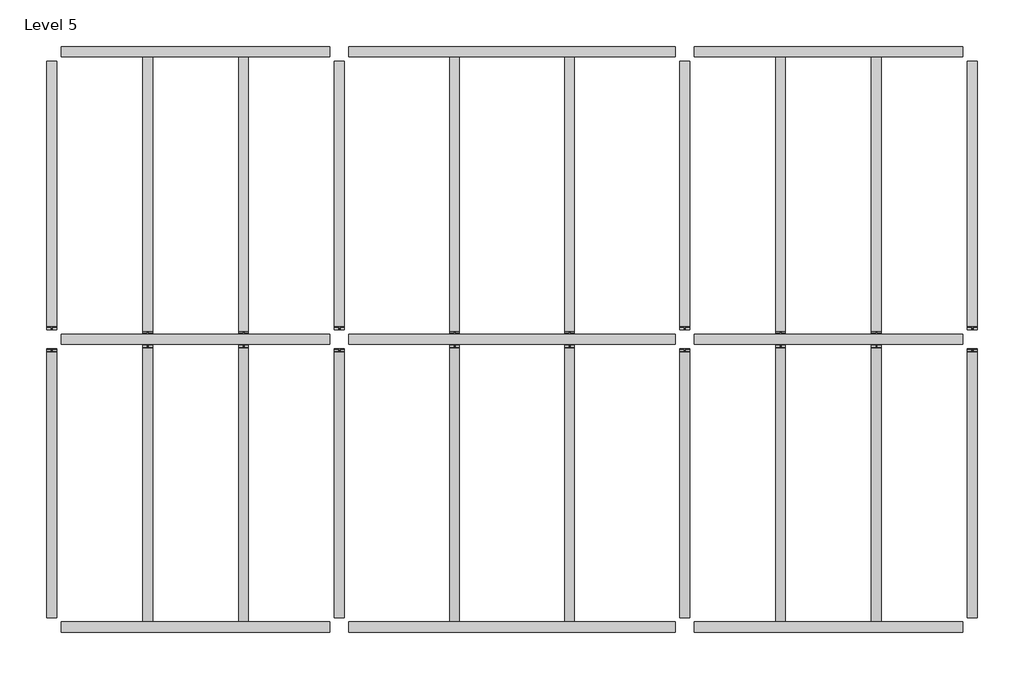
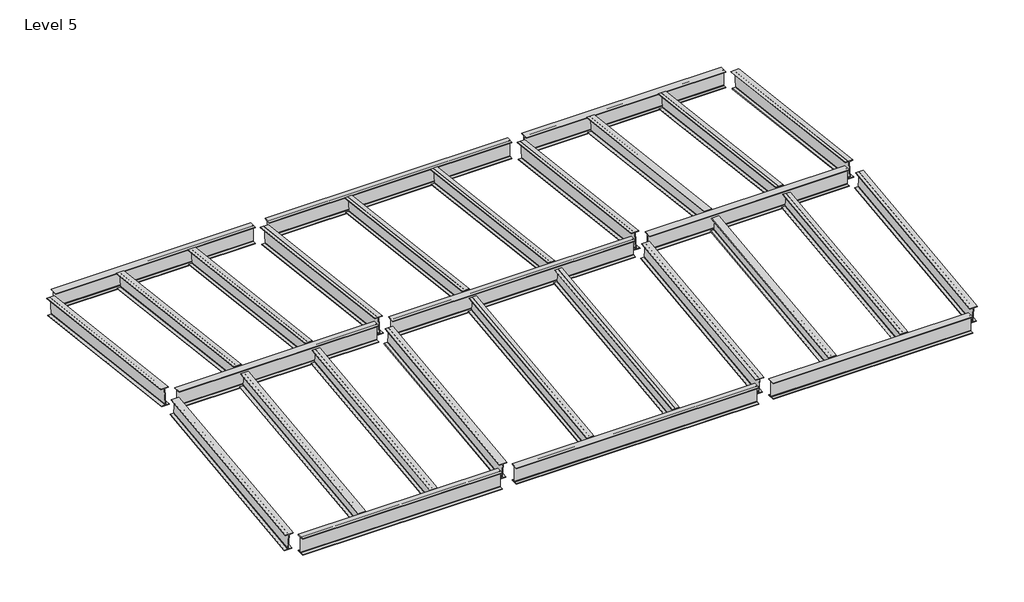
# One storey: 29 beams.
"""IFC4 building model written with IfcOpenShell, lengths in millimetres."""

import ifcopenshell
import ifcopenshell.guid

model = None  # the IFC model being written
_history = None  # IfcOwnerHistory: only IFC2X3 demands one
_inside = {}  # id of a spatial element -> (the spatial element, [elements in it])
_under = {}  # id of a project, library or spatial element -> (it, [spatial elements below it])
_declared = {}  # id of a project -> (the project, [libraries it declares])
_typed = {}  # id of a type object -> (the type object, [elements of that type])
_made_of = {}  # id of a material, layer set ... -> (it, [elements and type objects made of it])


def new_model(schema):
    """Start an empty IFC model of exactly this schema.

    Asked for "IFC4X3", IfcOpenShell would pick the latest addendum, in which some entities
    have other attributes; the version numbers below select the first issue.
    IFC2X3 requires an IfcOwnerHistory on every rooted entity: one is made here for all.
    """
    global model, _history
    if schema == "IFC4X3":
        model = ifcopenshell.file(schema_version=(4, 3, 0, 0))
    else:
        model = ifcopenshell.file(schema=schema)
    _inside.clear()
    _under.clear()
    _declared.clear()
    _typed.clear()
    _made_of.clear()
    _history = None
    if model.schema == "IFC2X3":
        org = make("IfcOrganization", Name="unknown")
        user = make(
            "IfcPersonAndOrganization",
            ThePerson=make("IfcPerson", FamilyName="unknown"),
            TheOrganization=org,
        )
        app = make(
            "IfcApplication",
            ApplicationDeveloper=org,
            Version="unknown",
            ApplicationFullName="unknown",
            ApplicationIdentifier="unknown",
        )
        _history = make(
            "IfcOwnerHistory",
            OwningUser=user,
            OwningApplication=app,
            ChangeAction="ADDED",
            CreationDate=0,
        )
    return model


def make(cls, **values):
    """One entity of the class cls with the attributes given. An attribute that is None is left unset."""
    return model.create_entity(
        cls, **{name: value for name, value in values.items() if value is not None}
    )


def rooted(cls, **values):
    """An entity with a GlobalId (a new one), such as an element, a storey or a relation."""
    return make(cls, GlobalId=ifcopenshell.guid.new(), OwnerHistory=_history, **values)


def si_unit(unit_type, name, prefix=None):
    """IfcSIUnit, for example si_unit("LENGTHUNIT", "METRE", prefix="MILLI")."""
    return make("IfcSIUnit", UnitType=unit_type, Prefix=prefix, Name=name)


def assignment(units):
    """IfcUnitAssignment: the units of a project."""
    return None if units is None else make("IfcUnitAssignment", Units=units)


def point(xyz):
    """IfcCartesianPoint."""
    return None if xyz is None else make("IfcCartesianPoint", Coordinates=xyz)


def direction(xyz):
    """IfcDirection."""
    return None if xyz is None else make("IfcDirection", DirectionRatios=xyz)


def frame(location, z_axis=None, x_axis=None):
    """IfcAxis2Placement3D, a coordinate frame: its origin and axes. An axis left out is left unset."""
    return make(
        "IfcAxis2Placement3D",
        Location=point(location),
        Axis=direction(z_axis),
        RefDirection=direction(x_axis),
    )


def frame_2d(location, x_axis=None):
    """IfcAxis2Placement2D, a coordinate frame in the plane: its origin and x axis."""
    return make(
        "IfcAxis2Placement2D", Location=point(location), RefDirection=direction(x_axis)
    )


def origin():
    """The frame at (0, 0, 0) with its axes left unset."""
    return frame((0.0, 0.0, 0.0))


def place(relative_to, where):
    """IfcLocalPlacement: puts the frame where relative to a parent placement (None: the world)."""
    return make(
        "IfcLocalPlacement", PlacementRelTo=relative_to, RelativePlacement=where
    )


def context(
    kind, dimensions, precision=None, world=None, true_north=None, identifier=None
):
    """IfcGeometricRepresentationContext, for example the 3D "Model" context."""
    return make(
        "IfcGeometricRepresentationContext",
        ContextIdentifier=identifier,
        ContextType=kind,
        CoordinateSpaceDimension=dimensions,
        Precision=precision,
        WorldCoordinateSystem=world,
        TrueNorth=true_north,
    )


def project(units=None, contexts=None):
    """IfcProject with its units and contexts."""
    return rooted(
        "IfcProject",
        Name="project",
        RepresentationContexts=contexts,
        UnitsInContext=assignment(units),
    )


def spatial(cls, under=None, at=None, **own):
    """A site, building, storey or space (cls), placed at a placement, below another one or the project."""
    s = rooted(cls, ObjectPlacement=at, **own)
    if under is not None:
        _under.setdefault(under.id(), (under, []))[1].append(s)
    return s


def polyline(points):
    """IfcPolyline through the points."""
    return make("IfcPolyline", Points=[point(p) for p in points])


def circle_curve(where, radius):
    """IfcCircle in the frame where."""
    return make("IfcCircle", Position=where, Radius=radius)


def trimmed(basis, trim1, trim2, sense, master):
    """IfcTrimmedCurve: the piece of a basis curve between two trims."""
    return make(
        "IfcTrimmedCurve",
        BasisCurve=basis,
        Trim1=trim1,
        Trim2=trim2,
        SenseAgreement=sense,
        MasterRepresentation=master,
    )


def segment(curve, same_sense, transition):
    """IfcCompositeCurveSegment."""
    return make(
        "IfcCompositeCurveSegment",
        Transition=transition,
        SameSense=same_sense,
        ParentCurve=curve,
    )


def composite_curve(segments, self_intersect=None):
    """IfcCompositeCurve: segments joined end to end."""
    return make("IfcCompositeCurve", Segments=segments, SelfIntersect=self_intersect)


def outline(outer, holes=None, kind="AREA"):
    """IfcArbitraryClosedProfileDef: a profile drawn as a closed curve; with holes, ...WithVoids."""
    if holes is None:
        return make("IfcArbitraryClosedProfileDef", ProfileType=kind, OuterCurve=outer)
    return make(
        "IfcArbitraryProfileDefWithVoids",
        ProfileType=kind,
        OuterCurve=outer,
        InnerCurves=holes,
    )


def extrude(swept, where, along, depth):
    """IfcExtrudedAreaSolid: the profile swept, set in the frame where, extruded along a direction by depth."""
    return make(
        "IfcExtrudedAreaSolid",
        SweptArea=swept,
        Position=where,
        ExtrudedDirection=direction(along),
        Depth=depth,
    )


def shape(context_of_items, identifier, shape_type, items):
    """IfcShapeRepresentation: the items that make up one representation, for example the "Body"."""
    return make(
        "IfcShapeRepresentation",
        ContextOfItems=context_of_items,
        RepresentationIdentifier=identifier,
        RepresentationType=shape_type,
        Items=items,
    )


def source(mapping_origin, context_of_items, identifier, shape_type, items):
    """IfcRepresentationMap: a shape defined once, which mapped items show again and again."""
    return make(
        "IfcRepresentationMap",
        MappingOrigin=mapping_origin,
        MappedRepresentation=shape(context_of_items, identifier, shape_type, items),
    )


def transform(
    local_origin,
    x_axis=None,
    y_axis=None,
    z_axis=None,
    scale=None,
    scale2=None,
    scale3=None,
    uniform=True,
):
    """IfcCartesianTransformationOperator3D, or its non-uniform kind. x_axis, y_axis, z_axis: its Axis1, 2, 3."""
    if uniform:
        return make(
            "IfcCartesianTransformationOperator3D",
            Axis1=direction(x_axis),
            Axis2=direction(y_axis),
            LocalOrigin=point(local_origin),
            Scale=scale,
            Axis3=direction(z_axis),
        )
    return make(
        "IfcCartesianTransformationOperator3DnonUniform",
        Axis1=direction(x_axis),
        Axis2=direction(y_axis),
        LocalOrigin=point(local_origin),
        Scale=scale,
        Axis3=direction(z_axis),
        Scale2=scale2,
        Scale3=scale3,
    )


def mapped(mapping_source, mapping_target):
    """IfcMappedItem: shows the shape of a source again, moved by a transform."""
    return make(
        "IfcMappedItem", MappingSource=mapping_source, MappingTarget=mapping_target
    )


def made_of(thing, what):
    """Note that an element or type object is made of a material, layer set ...; save() writes the relation."""
    if what is not None:
        _made_of.setdefault(what.id(), (what, []))[1].append(thing)
    return thing


def element(
    cls,
    number,
    at=None,
    inside=None,
    cuts=None,
    type_object=None,
    material=None,
    context=None,
    identifier="Body",
    shape_type=None,
    held_by="IfcProductDefinitionShape",
    body=None,
    shapes=None,
    **own,
):
    """One element of the class cls, such as IfcWall. Its Tag is "e" and its number.

    at: its placement. inside: the storey or other place that contains it. cuts: it is an
    opening in that element (IfcRelVoidsElement). A single representation is given by context,
    identifier, shape_type and body (its items); several are given by shapes. held_by: the class
    of the entity that holds the representations. save() writes the other relations.
    """
    e = rooted(cls, Tag="e%d" % number, ObjectPlacement=at, **own)
    if body is not None:
        shapes = [shape(context, identifier, shape_type, body)]
    if shapes is not None:
        e.Representation = make(held_by, Representations=shapes)
    if inside is not None:
        _inside.setdefault(inside.id(), (inside, []))[1].append(e)
    if cuts is not None:
        rooted(
            "IfcRelVoidsElement", RelatingBuildingElement=cuts, RelatedOpeningElement=e
        )
    if type_object is not None:
        _typed.setdefault(type_object.id(), (type_object, []))[1].append(e)
    return made_of(e, material)


def aggregate(whole, parts):
    """IfcRelAggregates: a whole, such as a stair, and the parts it consists of."""
    return rooted("IfcRelAggregates", RelatingObject=whole, RelatedObjects=parts)


def save(model, path):
    """Write the relations noted so far, then the file.

    IfcRelAggregates (storeys below a building ...), IfcRelContainedInSpatialStructure (elements
    in a storey), IfcRelDefinesByType, IfcRelAssociatesMaterial and IfcRelDeclares: one each for
    every whole, place, type object, material and project.
    """
    for whole, parts in _under.values():
        aggregate(whole, parts)
    for where, things in _inside.values():
        rooted(
            "IfcRelContainedInSpatialStructure",
            RelatedElements=things,
            RelatingStructure=where,
        )
    for kind, things in _typed.values():
        rooted("IfcRelDefinesByType", RelatedObjects=things, RelatingType=kind)
    for what, things in _made_of.values():
        rooted("IfcRelAssociatesMaterial", RelatedObjects=things, RelatingMaterial=what)
    for by, libraries in _declared.values():
        rooted("IfcRelDeclares", RelatingContext=by, RelatedDefinitions=libraries)
    model.write(path)


def ub_universal_beams_ub356x171x51_7273abb1(model_context):
    return source(origin(), model_context, "Body", "SweptSolid", [
        extrude(outline(composite_curve([segment(polyline([(85.75, -166.0), (85.75, -177.5), (-85.75, -177.5), (-85.75, -166.0), (-13.9, -166.0)]), True, "CONTINUOUS"), segment(trimmed(circle_curve(frame_2d((-13.9, -155.8)), 10.2), [point((-13.9, -166.0))], [point((-3.7, -155.8))], True, "CARTESIAN"), True, "CONTINUOUS"), segment(polyline([(-3.7, -155.8), (-3.7, 155.8)]), True, "CONTINUOUS"), segment(trimmed(circle_curve(frame_2d((-13.9, 155.8)), 10.2), [point((-3.7, 155.8))], [point((-13.9, 166.0))], True, "CARTESIAN"), True, "CONTINUOUS"), segment(polyline([(-13.9, 166.0), (-85.75, 166.0), (-85.75, 177.5), (85.75, 177.5), (85.75, 166.0), (13.9, 166.0)]), True, "CONTINUOUS"), segment(trimmed(circle_curve(frame_2d((13.9, 155.8)), 10.2), [point((13.9, 166.0))], [point((3.7, 155.8))], True, "CARTESIAN"), True, "CONTINUOUS"), segment(polyline([(3.7, 155.8), (3.7, -155.8)]), True, "CONTINUOUS"), segment(trimmed(circle_curve(frame_2d((13.9, -155.8)), 10.2), [point((3.7, -155.8))], [point((13.9, -166.0))], True, "CARTESIAN"), True, "CONTINUOUS"), segment(polyline([(13.9, -166.0), (85.75, -166.0)]), True, "CONTINUOUS")], self_intersect=False)), frame((-2416.9, 0.0, 0.0), z_axis=(1.0, 0.0, 0.0), x_axis=(0.0, 1.0, 0.0)), (0.0, 0.0, 1.0), 4789.9),
    ])


def ub_universal_beams_ub356x171x51_eaee8fc9(model_context):
    return source(origin(), model_context, "Body", "SweptSolid", [
        extrude(outline(composite_curve([segment(polyline([(85.75, -166.0), (85.75, -177.5), (-85.75, -177.5), (-85.75, -166.0), (-13.9, -166.0)]), True, "CONTINUOUS"), segment(trimmed(circle_curve(frame_2d((-13.9, -155.8)), 10.2), [point((-13.9, -166.0))], [point((-3.7, -155.8))], True, "CARTESIAN"), True, "CONTINUOUS"), segment(polyline([(-3.7, -155.8), (-3.7, 155.8)]), True, "CONTINUOUS"), segment(trimmed(circle_curve(frame_2d((-13.9, 155.8)), 10.2), [point((-3.7, 155.8))], [point((-13.9, 166.0))], True, "CARTESIAN"), True, "CONTINUOUS"), segment(polyline([(-13.9, 166.0), (-85.75, 166.0), (-85.75, 177.5), (85.75, 177.5), (85.75, 166.0), (13.9, 166.0)]), True, "CONTINUOUS"), segment(trimmed(circle_curve(frame_2d((13.9, 155.8)), 10.2), [point((13.9, 166.0))], [point((3.7, 155.8))], True, "CARTESIAN"), True, "CONTINUOUS"), segment(polyline([(3.7, 155.8), (3.7, -155.8)]), True, "CONTINUOUS"), segment(trimmed(circle_curve(frame_2d((13.9, -155.8)), 10.2), [point((3.7, -155.8))], [point((13.9, -166.0))], True, "CARTESIAN"), True, "CONTINUOUS"), segment(polyline([(13.9, -166.0), (85.75, -166.0)]), True, "CONTINUOUS")], self_intersect=False)), frame((-2373.0, 0.0, 0.0), z_axis=(1.0, 0.0, 0.0), x_axis=(0.0, 1.0, 0.0)), (0.0, 0.0, 1.0), 4789.9),
    ])


def ub_universal_beams_ub406x178x60_425a89a6(model_context):
    return source(origin(), model_context, "Body", "SweptSolid", [
        extrude(outline(composite_curve([segment(polyline([(88.95, -190.4), (88.95, -203.2), (-88.95, -203.2), (-88.95, -190.4), (-14.15, -190.4)]), True, "CONTINUOUS"), segment(trimmed(circle_curve(frame_2d((-14.15, -180.2)), 10.2), [point((-14.15, -190.4))], [point((-3.95, -180.2))], True, "CARTESIAN"), True, "CONTINUOUS"), segment(polyline([(-3.95, -180.2), (-3.95, 180.2)]), True, "CONTINUOUS"), segment(trimmed(circle_curve(frame_2d((-14.15, 180.2)), 10.2), [point((-3.95, 180.2))], [point((-14.15, 190.4))], True, "CARTESIAN"), True, "CONTINUOUS"), segment(polyline([(-14.15, 190.4), (-88.95, 190.4), (-88.95, 203.2), (88.95, 203.2), (88.95, 190.4), (14.15, 190.4)]), True, "CONTINUOUS"), segment(trimmed(circle_curve(frame_2d((14.15, 180.2)), 10.2), [point((14.15, 190.4))], [point((3.95, 180.2))], True, "CARTESIAN"), True, "CONTINUOUS"), segment(polyline([(3.95, 180.2), (3.95, -180.2)]), True, "CONTINUOUS"), segment(trimmed(circle_curve(frame_2d((14.15, -180.2)), 10.2), [point((3.95, -180.2))], [point((14.15, -190.4))], True, "CARTESIAN"), True, "CONTINUOUS"), segment(polyline([(14.15, -190.4), (88.95, -190.4)]), True, "CONTINUOUS")], self_intersect=False)), frame((-2334.6, 0.0, 0.0), z_axis=(1.0, 0.0, 0.0), x_axis=(0.0, 1.0, 0.0)), (0.0, 0.0, 1.0), 4669.2),
    ])


def ub_universal_beams_ub406x178x60_ab0c7e2f(model_context):
    return source(origin(), model_context, "Body", "SweptSolid", [
        extrude(outline(composite_curve([segment(polyline([(88.95, -190.4), (88.95, -203.2), (-88.95, -203.2), (-88.95, -190.4), (-14.15, -190.4)]), True, "CONTINUOUS"), segment(trimmed(circle_curve(frame_2d((-14.15, -180.2)), 10.2), [point((-14.15, -190.4))], [point((-3.95, -180.2))], True, "CARTESIAN"), True, "CONTINUOUS"), segment(polyline([(-3.95, -180.2), (-3.95, 180.2)]), True, "CONTINUOUS"), segment(trimmed(circle_curve(frame_2d((-14.15, 180.2)), 10.2), [point((-3.95, 180.2))], [point((-14.15, 190.4))], True, "CARTESIAN"), True, "CONTINUOUS"), segment(polyline([(-14.15, 190.4), (-88.95, 190.4), (-88.95, 203.2), (88.95, 203.2), (88.95, 190.4), (14.15, 190.4)]), True, "CONTINUOUS"), segment(trimmed(circle_curve(frame_2d((14.15, 180.2)), 10.2), [point((14.15, 190.4))], [point((3.95, 180.2))], True, "CARTESIAN"), True, "CONTINUOUS"), segment(polyline([(3.95, 180.2), (3.95, -180.2)]), True, "CONTINUOUS"), segment(trimmed(circle_curve(frame_2d((14.15, -180.2)), 10.2), [point((3.95, -180.2))], [point((14.15, -190.4))], True, "CARTESIAN"), True, "CONTINUOUS"), segment(polyline([(14.15, -190.4), (88.95, -190.4)]), True, "CONTINUOUS")], self_intersect=False)), frame((-2834.6, 0.0, 0.0), z_axis=(1.0, 0.0, 0.0), x_axis=(0.0, 1.0, 0.0)), (0.0, 0.0, 1.0), 5669.2),
    ])


def ub_universal_beams_ub406x178x60_0db8b4c4(model_context):
    return source(origin(), model_context, "Body", "SweptSolid", [
        extrude(outline(composite_curve([segment(polyline([(88.95, -190.4), (88.95, -203.2), (-88.95, -203.2), (-88.95, -190.4), (-14.15, -190.4)]), True, "CONTINUOUS"), segment(trimmed(circle_curve(frame_2d((-14.15, -180.2)), 10.2), [point((-14.15, -190.4))], [point((-3.95, -180.2))], True, "CARTESIAN"), True, "CONTINUOUS"), segment(polyline([(-3.95, -180.2), (-3.95, 180.2)]), True, "CONTINUOUS"), segment(trimmed(circle_curve(frame_2d((-14.15, 180.2)), 10.2), [point((-3.95, 180.2))], [point((-14.15, 190.4))], True, "CARTESIAN"), True, "CONTINUOUS"), segment(polyline([(-14.15, 190.4), (-88.95, 190.4), (-88.95, 203.2), (88.95, 203.2), (88.95, 190.4), (14.15, 190.4)]), True, "CONTINUOUS"), segment(trimmed(circle_curve(frame_2d((14.15, 180.2)), 10.2), [point((14.15, 190.4))], [point((3.95, 180.2))], True, "CARTESIAN"), True, "CONTINUOUS"), segment(polyline([(3.95, 180.2), (3.95, -180.2)]), True, "CONTINUOUS"), segment(trimmed(circle_curve(frame_2d((14.15, -180.2)), 10.2), [point((3.95, -180.2))], [point((14.15, -190.4))], True, "CARTESIAN"), True, "CONTINUOUS"), segment(polyline([(14.15, -190.4), (88.95, -190.4)]), True, "CONTINUOUS")], self_intersect=False)), frame((-2352.35, 0.0, 0.0), z_axis=(1.0, 0.0, 0.0), x_axis=(0.0, 1.0, 0.0)), (0.0, 0.0, 1.0), 4653.7),
    ])


def ub_universal_beams_ub406x178x60_0ea3e6ef(model_context):
    return source(origin(), model_context, "Body", "SweptSolid", [
        extrude(outline(composite_curve([segment(polyline([(88.95, -190.4), (88.95, -203.2), (-88.95, -203.2), (-88.95, -190.4), (-14.15, -190.4)]), True, "CONTINUOUS"), segment(trimmed(circle_curve(frame_2d((-14.15, -180.2)), 10.2), [point((-14.15, -190.4))], [point((-3.95, -180.2))], True, "CARTESIAN"), True, "CONTINUOUS"), segment(polyline([(-3.95, -180.2), (-3.95, 180.2)]), True, "CONTINUOUS"), segment(trimmed(circle_curve(frame_2d((-14.15, 180.2)), 10.2), [point((-3.95, 180.2))], [point((-14.15, 190.4))], True, "CARTESIAN"), True, "CONTINUOUS"), segment(polyline([(-14.15, 190.4), (-88.95, 190.4), (-88.95, 203.2), (88.95, 203.2), (88.95, 190.4), (14.15, 190.4)]), True, "CONTINUOUS"), segment(trimmed(circle_curve(frame_2d((14.15, 180.2)), 10.2), [point((14.15, 190.4))], [point((3.95, 180.2))], True, "CARTESIAN"), True, "CONTINUOUS"), segment(polyline([(3.95, 180.2), (3.95, -180.2)]), True, "CONTINUOUS"), segment(trimmed(circle_curve(frame_2d((14.15, -180.2)), 10.2), [point((3.95, -180.2))], [point((14.15, -190.4))], True, "CARTESIAN"), True, "CONTINUOUS"), segment(polyline([(14.15, -190.4), (88.95, -190.4)]), True, "CONTINUOUS")], self_intersect=False)), frame((-2301.35, 0.0, 0.0), z_axis=(1.0, 0.0, 0.0), x_axis=(0.0, 1.0, 0.0)), (0.0, 0.0, 1.0), 4653.7),
    ])


model = new_model("IFC4")

# Units and contexts
model_context = context("Model", 3, world=origin())
ifc_project = project(units=[si_unit("LENGTHUNIT", "METRE", prefix="MILLI")], contexts=[model_context])

# Site, building, storey
site = spatial("IfcSite", under=ifc_project)
building = spatial("IfcBuilding", under=site)
storey = spatial("IfcBuildingStorey", under=building, Name="Level 5", Elevation=12500.0)

# Beams
placement = place(None, origin())
ub_universal_beams_ub356x171x51_shape = ub_universal_beams_ub356x171x51_7273abb1(model_context)
element("IfcBeam", 1, ObjectType="UB-Universal Beams : UB356x171x51", at=placement, inside=storey, context=model_context, shape_type="MappedRepresentation", body=[
    mapped(ub_universal_beams_ub356x171x51_shape, transform((1666.6666667, 2521.1482767, 12623.7643612), x_axis=(0.0, 0.992876838486922, 0.11914522061843107), y_axis=(-1.0, 0.0, 0.0), z_axis=(0.0, -0.11914522061843107, 0.992876838486922))),
])
element("IfcBeam", 2, ObjectType="UB-Universal Beams : UB356x171x51", at=placement, inside=storey, context=model_context, shape_type="MappedRepresentation", body=[
    mapped(ub_universal_beams_ub356x171x51_shape, transform((3333.3333333, 2521.1482767, 12623.7643612), x_axis=(0.0, 0.992876838486922, 0.11914522061843107), y_axis=(-1.0, 0.0, 0.0), z_axis=(0.0, -0.11914522061843107, 0.992876838486922))),
])
element("IfcBeam", 3, ObjectType="UB-Universal Beams : UB356x171x51", at=placement, inside=storey, context=model_context, shape_type="MappedRepresentation", body=[
    mapped(ub_universal_beams_ub356x171x51_shape, transform((7000.0, 2521.1482767, 12623.7643612), x_axis=(0.0, 0.992876838486922, 0.11914522061843107), y_axis=(-1.0, 0.0, 0.0), z_axis=(0.0, -0.11914522061843107, 0.992876838486922))),
])
element("IfcBeam", 4, ObjectType="UB-Universal Beams : UB356x171x51", at=placement, inside=storey, context=model_context, shape_type="MappedRepresentation", body=[
    mapped(ub_universal_beams_ub356x171x51_shape, transform((9000.0, 2521.1482767, 12623.7643612), x_axis=(0.0, 0.992876838486922, 0.11914522061843107), y_axis=(-1.0, 0.0, 0.0), z_axis=(0.0, -0.11914522061843107, 0.992876838486922))),
])
element("IfcBeam", 5, ObjectType="UB-Universal Beams : UB356x171x51", at=placement, inside=storey, context=model_context, shape_type="MappedRepresentation", body=[
    mapped(ub_universal_beams_ub356x171x51_shape, transform((12666.6666667, 2521.1482767, 12623.7643612), x_axis=(0.0, 0.992876838486922, 0.11914522061843107), y_axis=(-1.0, 0.0, 0.0), z_axis=(0.0, -0.11914522061843107, 0.992876838486922))),
])
element("IfcBeam", 6, ObjectType="UB-Universal Beams : UB356x171x51", at=placement, inside=storey, context=model_context, shape_type="MappedRepresentation", body=[
    mapped(ub_universal_beams_ub356x171x51_shape, transform((14333.3333333, 2521.1482767, 12623.7643612), x_axis=(0.0, 0.992876838486922, 0.11914522061843107), y_axis=(-1.0, 0.0, 0.0), z_axis=(0.0, -0.11914522061843107, 0.992876838486922))),
])
ub_universal_beams_ub356x171x51_2_shape = ub_universal_beams_ub356x171x51_eaee8fc9(model_context)
element("IfcBeam", 7, ObjectType="UB-Universal Beams : UB356x171x51", at=placement, inside=storey, context=model_context, shape_type="MappedRepresentation", body=[
    mapped(ub_universal_beams_ub356x171x51_2_shape, transform((1666.6666667, 7478.8517233, 12623.7643612), x_axis=(0.0, 0.992876838486922, -0.11914522061843064), y_axis=(-1.0, 0.0, 0.0), z_axis=(0.0, 0.11914522061843062, 0.9928768384869221))),
])
element("IfcBeam", 8, ObjectType="UB-Universal Beams : UB356x171x51", at=placement, inside=storey, context=model_context, shape_type="MappedRepresentation", body=[
    mapped(ub_universal_beams_ub356x171x51_2_shape, transform((3333.3333333, 7478.8517233, 12623.7643612), x_axis=(0.0, 0.992876838486922, -0.11914522061843064), y_axis=(-1.0, 0.0, 0.0), z_axis=(0.0, 0.11914522061843062, 0.9928768384869221))),
])
element("IfcBeam", 9, ObjectType="UB-Universal Beams : UB356x171x51", at=placement, inside=storey, context=model_context, shape_type="MappedRepresentation", body=[
    mapped(ub_universal_beams_ub356x171x51_2_shape, transform((7000.0, 7478.8517233, 12623.7643612), x_axis=(0.0, 0.992876838486922, -0.11914522061843064), y_axis=(-1.0, 0.0, 0.0), z_axis=(0.0, 0.11914522061843062, 0.9928768384869221))),
])
element("IfcBeam", 10, ObjectType="UB-Universal Beams : UB356x171x51", at=placement, inside=storey, context=model_context, shape_type="MappedRepresentation", body=[
    mapped(ub_universal_beams_ub356x171x51_2_shape, transform((9000.0, 7478.8517233, 12623.7643612), x_axis=(0.0, 0.992876838486922, -0.11914522061843064), y_axis=(-1.0, 0.0, 0.0), z_axis=(0.0, 0.11914522061843062, 0.9928768384869221))),
])
element("IfcBeam", 11, ObjectType="UB-Universal Beams : UB356x171x51", at=placement, inside=storey, context=model_context, shape_type="MappedRepresentation", body=[
    mapped(ub_universal_beams_ub356x171x51_2_shape, transform((12666.6666667, 7478.8517233, 12623.7643612), x_axis=(0.0, 0.992876838486922, -0.11914522061843064), y_axis=(-1.0, 0.0, 0.0), z_axis=(0.0, 0.11914522061843062, 0.9928768384869221))),
])
element("IfcBeam", 12, ObjectType="UB-Universal Beams : UB356x171x51", at=placement, inside=storey, context=model_context, shape_type="MappedRepresentation", body=[
    mapped(ub_universal_beams_ub356x171x51_2_shape, transform((14333.3333333, 7478.8517233, 12623.7643612), x_axis=(0.0, 0.992876838486922, -0.11914522061843064), y_axis=(-1.0, 0.0, 0.0), z_axis=(0.0, 0.11914522061843062, 0.9928768384869221))),
])
ub_universal_beams_ub406x178x60_shape = ub_universal_beams_ub406x178x60_425a89a6(model_context)
element("IfcBeam", 13, ObjectType="UB-Universal Beams : UB406x178x60", at=placement, inside=storey, context=model_context, shape_type="MappedRepresentation", body=[
    mapped(ub_universal_beams_ub406x178x60_shape, transform((2500.0, 0.0, 12296.8), x_axis=(1.0, 0.0, 0.0), y_axis=(0.0, 1.0, 0.0), z_axis=(0.0, 0.0, 1.0))),
])
element("IfcBeam", 14, ObjectType="UB-Universal Beams : UB406x178x60", at=placement, inside=storey, context=model_context, shape_type="MappedRepresentation", body=[
    mapped(ub_universal_beams_ub406x178x60_shape, transform((13500.0, 0.0, 12296.8), x_axis=(1.0, 0.0, 0.0), y_axis=(0.0, 1.0, 0.0), z_axis=(0.0, 0.0, 1.0))),
])
element("IfcBeam", 15, ObjectType="UB-Universal Beams : UB406x178x60", at=placement, inside=storey, context=model_context, shape_type="MappedRepresentation", body=[
    mapped(ub_universal_beams_ub406x178x60_shape, transform((2500.0, 5000.0, 12896.8), x_axis=(1.0, 0.0, 0.0), y_axis=(0.0, 1.0, 0.0), z_axis=(0.0, 0.0, 1.0))),
])
element("IfcBeam", 16, ObjectType="UB-Universal Beams : UB406x178x60", at=placement, inside=storey, context=model_context, shape_type="MappedRepresentation", body=[
    mapped(ub_universal_beams_ub406x178x60_shape, transform((13500.0, 5000.0, 12896.8), x_axis=(1.0, 0.0, 0.0), y_axis=(0.0, 1.0, 0.0), z_axis=(0.0, 0.0, 1.0))),
])
element("IfcBeam", 17, ObjectType="UB-Universal Beams : UB406x178x60", at=placement, inside=storey, context=model_context, shape_type="MappedRepresentation", body=[
    mapped(ub_universal_beams_ub406x178x60_shape, transform((2500.0, 10000.0, 12296.8), x_axis=(1.0, 0.0, 0.0), y_axis=(0.0, 1.0, 0.0), z_axis=(0.0, 0.0, 1.0))),
])
element("IfcBeam", 18, ObjectType="UB-Universal Beams : UB406x178x60", at=placement, inside=storey, context=model_context, shape_type="MappedRepresentation", body=[
    mapped(ub_universal_beams_ub406x178x60_shape, transform((13500.0, 10000.0, 12296.8), x_axis=(1.0, 0.0, 0.0), y_axis=(0.0, 1.0, 0.0), z_axis=(0.0, 0.0, 1.0))),
])
ub_universal_beams_ub406x178x60_2_shape = ub_universal_beams_ub406x178x60_ab0c7e2f(model_context)
element("IfcBeam", 19, ObjectType="UB-Universal Beams : UB406x178x60", at=placement, inside=storey, context=model_context, shape_type="MappedRepresentation", body=[
    mapped(ub_universal_beams_ub406x178x60_2_shape, transform((8000.0, 0.0, 12296.8), x_axis=(1.0, 0.0, 0.0), y_axis=(0.0, 1.0, 0.0), z_axis=(0.0, 0.0, 1.0))),
])
element("IfcBeam", 20, ObjectType="UB-Universal Beams : UB406x178x60", at=placement, inside=storey, context=model_context, shape_type="MappedRepresentation", body=[
    mapped(ub_universal_beams_ub406x178x60_2_shape, transform((8000.0, 5000.0, 12896.8), x_axis=(1.0, 0.0, 0.0), y_axis=(0.0, 1.0, 0.0), z_axis=(0.0, 0.0, 1.0))),
])
element("IfcBeam", 21, ObjectType="UB-Universal Beams : UB406x178x60", at=placement, inside=storey, context=model_context, shape_type="MappedRepresentation", body=[
    mapped(ub_universal_beams_ub406x178x60_2_shape, transform((8000.0, 10000.0, 12296.8), x_axis=(1.0, 0.0, 0.0), y_axis=(0.0, 1.0, 0.0), z_axis=(0.0, 0.0, 1.0))),
])
ub_universal_beams_ub406x178x60_3_shape = ub_universal_beams_ub406x178x60_0db8b4c4(model_context)
element("IfcBeam", 22, ObjectType="UB-Universal Beams : UB406x178x60", at=placement, inside=storey, context=model_context, shape_type="MappedRepresentation", body=[
    mapped(ub_universal_beams_ub406x178x60_3_shape, transform((0.0, 2524.2103088, 12598.2474264), x_axis=(0.0, 0.992876838486922, 0.11914522061843107), y_axis=(-1.0, 0.0, 0.0), z_axis=(0.0, -0.11914522061843107, 0.992876838486922))),
])
element("IfcBeam", 23, ObjectType="UB-Universal Beams : UB406x178x60", at=placement, inside=storey, context=model_context, shape_type="MappedRepresentation", body=[
    mapped(ub_universal_beams_ub406x178x60_3_shape, transform((5000.0, 2524.2103088, 12598.2474264), x_axis=(0.0, 0.992876838486922, 0.11914522061843107), y_axis=(-1.0, 0.0, 0.0), z_axis=(0.0, -0.11914522061843107, 0.992876838486922))),
])
element("IfcBeam", 24, ObjectType="UB-Universal Beams : UB406x178x60", at=placement, inside=storey, context=model_context, shape_type="MappedRepresentation", body=[
    mapped(ub_universal_beams_ub406x178x60_3_shape, transform((11000.0, 2524.2103088, 12598.2474264), x_axis=(0.0, 0.992876838486922, 0.11914522061843107), y_axis=(-1.0, 0.0, 0.0), z_axis=(0.0, -0.11914522061843107, 0.992876838486922))),
])
element("IfcBeam", 25, ObjectType="UB-Universal Beams : UB406x178x60", at=placement, inside=storey, context=model_context, shape_type="MappedRepresentation", body=[
    mapped(ub_universal_beams_ub406x178x60_3_shape, transform((16000.0, 2524.2103088, 12598.2474264), x_axis=(0.0, 0.992876838486922, 0.11914522061843107), y_axis=(-1.0, 0.0, 0.0), z_axis=(0.0, -0.11914522061843107, 0.992876838486922))),
])
ub_universal_beams_ub406x178x60_4_shape = ub_universal_beams_ub406x178x60_0ea3e6ef(model_context)
element("IfcBeam", 26, ObjectType="UB-Universal Beams : UB406x178x60", at=placement, inside=storey, context=model_context, shape_type="MappedRepresentation", body=[
    mapped(ub_universal_beams_ub406x178x60_4_shape, transform((0.0, 7475.7896912, 12598.2474264), x_axis=(0.0, 0.992876838486922, -0.11914522061843064), y_axis=(-1.0, 0.0, 0.0), z_axis=(0.0, 0.11914522061843062, 0.9928768384869221))),
])
element("IfcBeam", 27, ObjectType="UB-Universal Beams : UB406x178x60", at=placement, inside=storey, context=model_context, shape_type="MappedRepresentation", body=[
    mapped(ub_universal_beams_ub406x178x60_4_shape, transform((5000.0, 7475.7896912, 12598.2474264), x_axis=(0.0, 0.992876838486922, -0.11914522061843064), y_axis=(-1.0, 0.0, 0.0), z_axis=(0.0, 0.11914522061843062, 0.9928768384869221))),
])
element("IfcBeam", 28, ObjectType="UB-Universal Beams : UB406x178x60", at=placement, inside=storey, context=model_context, shape_type="MappedRepresentation", body=[
    mapped(ub_universal_beams_ub406x178x60_4_shape, transform((11000.0, 7475.7896912, 12598.2474264), x_axis=(0.0, 0.992876838486922, -0.11914522061843064), y_axis=(-1.0, 0.0, 0.0), z_axis=(0.0, 0.11914522061843062, 0.9928768384869221))),
])
element("IfcBeam", 29, ObjectType="UB-Universal Beams : UB406x178x60", at=placement, inside=storey, context=model_context, shape_type="MappedRepresentation", body=[
    mapped(ub_universal_beams_ub406x178x60_4_shape, transform((16000.0, 7475.7896912, 12598.2474264), x_axis=(0.0, 0.992876838486922, -0.11914522061843064), y_axis=(-1.0, 0.0, 0.0), z_axis=(0.0, 0.11914522061843062, 0.9928768384869221))),
])

save(model, "model.ifc")

# Revit data of these elements
# Type "UB-Universal Beams : UB356x171x51"
#   Section Name Key = "UB356X171X51"
#   Width = 17.15 cm
#   Web Thickness = 0.74 cm
#   Web Fillet = 1.02 cm
#   Warping Constant = 286000.0 cm⁶
#   Torsional Moment of Inertia = 23.80 cm⁴
#   Section Area = 64.9 cm²
#   Plastic Modulus weak axis = 174.0 cm³
#   Plastic Modulus strong axis = 896.0 cm³
#   Nominal Weight = 50.9998 kgf/m
#   Moment of Inertia weak axis = 968.00 cm⁴
#   Moment of Inertia strong axis = 14136.00 cm⁴
#   Height = 35.5 cm
#   Flange Thickness = 1.15 cm
#   Elastic Modulus weak axis = 113.0 cm³
#   Elastic Modulus strong axis = 796.0 cm³
#   Centroid Vertical = 17.75 cm
#   Centroid Horizontal = 8.575 cm
#   Bolt Spacing = 9.0 cm
#   Length [instance default] = 1500 mm
#   Structural Material [instance default] = Metal - Steel 43-275
#   Type Comments = ""
#   Assembly Code = ""
# Type "UB-Universal Beams : UB406x178x60"
#   Section Name Key = "UB406X178X60"
#   Width = 17.79 cm
#   Web Thickness = 0.79 cm
#   Web Fillet = 1.02 cm
#   Warping Constant = 466000.0 cm⁶
#   Torsional Moment of Inertia = 33.30 cm⁴
#   Section Area = 76.5 cm²
#   Plastic Modulus weak axis = 209.0 cm³
#   Plastic Modulus strong axis = 1200.0 cm³
#   Nominal Weight = 60.0998 kgf/m
#   Moment of Inertia weak axis = 1203.00 cm⁴
#   Moment of Inertia strong axis = 21596.00 cm⁴
#   Height = 40.64 cm
#   Flange Thickness = 1.28 cm
#   Elastic Modulus weak axis = 135.0 cm³
#   Elastic Modulus strong axis = 1063.0 cm³
#   Centroid Vertical = 20.32 cm
#   Centroid Horizontal = 8.895 cm
#   Bolt Spacing = 9.0 cm
#   Length [instance default] = 1500 mm
#   Structural Material [instance default] = Metal - Steel 43-275
#   Type Comments = ""
#   Assembly Code = ""
# Elements 1, 2, 3, 4, 5, 6, 7, 8, 9, 10, 11, 12 (IfcBeam, "UB-Universal Beams : UB356x171x51")
#   Structural Material = Metal - Steel 43-275
#   Phase Created = New Construction
#   Materials on its faces: "Metal - Steel 43-275"
# Elements 13, 14, 15, 16, 17, 18, 19, 20, 21, 22, 23, 24, 25, 26, 27, 28, 29 (IfcBeam, "UB-Universal Beams : UB406x178x60")
#   Structural Material = Metal - Steel 43-275
#   Phase Created = New Construction
#   Materials on its faces: "Metal - Steel 43-275"
# Materials
#   "Metal - Steel 43-275": class "Metal", colour RGB 247 247 247, transparency 0, Cost = 0
